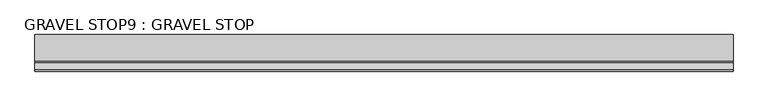
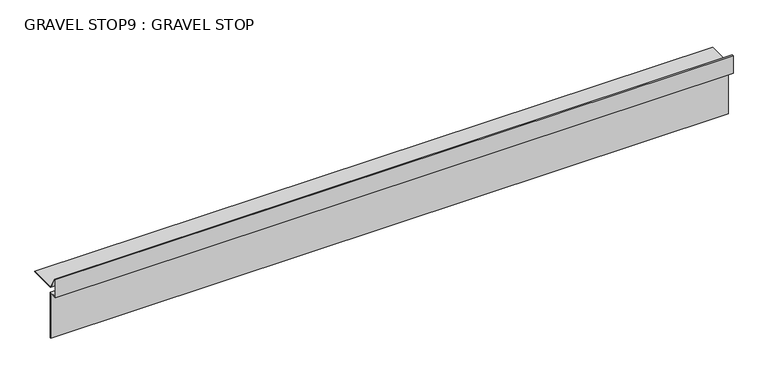
"""IFC4 building model written with IfcOpenShell, lengths in millimetres: proxy geometry, GRAVEL STOP9 : GRAVEL STOP."""

import ifcopenshell
import ifcopenshell.guid

model = None  # the IFC model being written
_history = None  # IfcOwnerHistory: only IFC2X3 demands one
_inside = {}  # id of a spatial element -> (the spatial element, [elements in it])
_under = {}  # id of a project, library or spatial element -> (it, [spatial elements below it])
_declared = {}  # id of a project -> (the project, [libraries it declares])
_typed = {}  # id of a type object -> (the type object, [elements of that type])
_made_of = {}  # id of a material, layer set ... -> (it, [elements and type objects made of it])


def new_model(schema):
    """Start an empty IFC model of exactly this schema.

    Asked for "IFC4X3", IfcOpenShell would pick the latest addendum, in which some entities
    have other attributes; the version numbers below select the first issue.
    IFC2X3 requires an IfcOwnerHistory on every rooted entity: one is made here for all.
    """
    global model, _history
    if schema == "IFC4X3":
        model = ifcopenshell.file(schema_version=(4, 3, 0, 0))
    else:
        model = ifcopenshell.file(schema=schema)
    _inside.clear()
    _under.clear()
    _declared.clear()
    _typed.clear()
    _made_of.clear()
    _history = None
    if model.schema == "IFC2X3":
        org = make("IfcOrganization", Name="unknown")
        user = make(
            "IfcPersonAndOrganization",
            ThePerson=make("IfcPerson", FamilyName="unknown"),
            TheOrganization=org,
        )
        app = make(
            "IfcApplication",
            ApplicationDeveloper=org,
            Version="unknown",
            ApplicationFullName="unknown",
            ApplicationIdentifier="unknown",
        )
        _history = make(
            "IfcOwnerHistory",
            OwningUser=user,
            OwningApplication=app,
            ChangeAction="ADDED",
            CreationDate=0,
        )
    return model


def make(cls, **values):
    """One entity of the class cls with the attributes given. An attribute that is None is left unset."""
    return model.create_entity(
        cls, **{name: value for name, value in values.items() if value is not None}
    )


def rooted(cls, **values):
    """An entity with a GlobalId (a new one), such as an element, a storey or a relation."""
    return make(cls, GlobalId=ifcopenshell.guid.new(), OwnerHistory=_history, **values)


def si_unit(unit_type, name, prefix=None):
    """IfcSIUnit, for example si_unit("LENGTHUNIT", "METRE", prefix="MILLI")."""
    return make("IfcSIUnit", UnitType=unit_type, Prefix=prefix, Name=name)


def assignment(units):
    """IfcUnitAssignment: the units of a project."""
    return None if units is None else make("IfcUnitAssignment", Units=units)


def point(xyz):
    """IfcCartesianPoint."""
    return None if xyz is None else make("IfcCartesianPoint", Coordinates=xyz)


def direction(xyz):
    """IfcDirection."""
    return None if xyz is None else make("IfcDirection", DirectionRatios=xyz)


def frame(location, z_axis=None, x_axis=None):
    """IfcAxis2Placement3D, a coordinate frame: its origin and axes. An axis left out is left unset."""
    return make(
        "IfcAxis2Placement3D",
        Location=point(location),
        Axis=direction(z_axis),
        RefDirection=direction(x_axis),
    )


def origin():
    """The frame at (0, 0, 0) with its axes left unset."""
    return frame((0.0, 0.0, 0.0))


def place(relative_to, where):
    """IfcLocalPlacement: puts the frame where relative to a parent placement (None: the world)."""
    return make(
        "IfcLocalPlacement", PlacementRelTo=relative_to, RelativePlacement=where
    )


def context(
    kind, dimensions, precision=None, world=None, true_north=None, identifier=None
):
    """IfcGeometricRepresentationContext, for example the 3D "Model" context."""
    return make(
        "IfcGeometricRepresentationContext",
        ContextIdentifier=identifier,
        ContextType=kind,
        CoordinateSpaceDimension=dimensions,
        Precision=precision,
        WorldCoordinateSystem=world,
        TrueNorth=true_north,
    )


def project(units=None, contexts=None):
    """IfcProject with its units and contexts."""
    return rooted(
        "IfcProject",
        Name="project",
        RepresentationContexts=contexts,
        UnitsInContext=assignment(units),
    )


def spatial(cls, under=None, at=None, **own):
    """A site, building, storey or space (cls), placed at a placement, below another one or the project."""
    s = rooted(cls, ObjectPlacement=at, **own)
    if under is not None:
        _under.setdefault(under.id(), (under, []))[1].append(s)
    return s


def polyline(points):
    """IfcPolyline through the points."""
    return make("IfcPolyline", Points=[point(p) for p in points])


def outline(outer, holes=None, kind="AREA"):
    """IfcArbitraryClosedProfileDef: a profile drawn as a closed curve; with holes, ...WithVoids."""
    if holes is None:
        return make("IfcArbitraryClosedProfileDef", ProfileType=kind, OuterCurve=outer)
    return make(
        "IfcArbitraryProfileDefWithVoids",
        ProfileType=kind,
        OuterCurve=outer,
        InnerCurves=holes,
    )


def extrude(swept, where, along, depth):
    """IfcExtrudedAreaSolid: the profile swept, set in the frame where, extruded along a direction by depth."""
    return make(
        "IfcExtrudedAreaSolid",
        SweptArea=swept,
        Position=where,
        ExtrudedDirection=direction(along),
        Depth=depth,
    )


def shape(context_of_items, identifier, shape_type, items):
    """IfcShapeRepresentation: the items that make up one representation, for example the "Body"."""
    return make(
        "IfcShapeRepresentation",
        ContextOfItems=context_of_items,
        RepresentationIdentifier=identifier,
        RepresentationType=shape_type,
        Items=items,
    )


def source(mapping_origin, context_of_items, identifier, shape_type, items):
    """IfcRepresentationMap: a shape defined once, which mapped items show again and again."""
    return make(
        "IfcRepresentationMap",
        MappingOrigin=mapping_origin,
        MappedRepresentation=shape(context_of_items, identifier, shape_type, items),
    )


def transform(
    local_origin,
    x_axis=None,
    y_axis=None,
    z_axis=None,
    scale=None,
    scale2=None,
    scale3=None,
    uniform=True,
):
    """IfcCartesianTransformationOperator3D, or its non-uniform kind. x_axis, y_axis, z_axis: its Axis1, 2, 3."""
    if uniform:
        return make(
            "IfcCartesianTransformationOperator3D",
            Axis1=direction(x_axis),
            Axis2=direction(y_axis),
            LocalOrigin=point(local_origin),
            Scale=scale,
            Axis3=direction(z_axis),
        )
    return make(
        "IfcCartesianTransformationOperator3DnonUniform",
        Axis1=direction(x_axis),
        Axis2=direction(y_axis),
        LocalOrigin=point(local_origin),
        Scale=scale,
        Axis3=direction(z_axis),
        Scale2=scale2,
        Scale3=scale3,
    )


def mapped(mapping_source, mapping_target):
    """IfcMappedItem: shows the shape of a source again, moved by a transform."""
    return make(
        "IfcMappedItem", MappingSource=mapping_source, MappingTarget=mapping_target
    )


def made_of(thing, what):
    """Note that an element or type object is made of a material, layer set ...; save() writes the relation."""
    if what is not None:
        _made_of.setdefault(what.id(), (what, []))[1].append(thing)
    return thing


def element(
    cls,
    number,
    at=None,
    inside=None,
    cuts=None,
    type_object=None,
    material=None,
    context=None,
    identifier="Body",
    shape_type=None,
    held_by="IfcProductDefinitionShape",
    body=None,
    shapes=None,
    **own,
):
    """One element of the class cls, such as IfcWall. Its Tag is "e" and its number.

    at: its placement. inside: the storey or other place that contains it. cuts: it is an
    opening in that element (IfcRelVoidsElement). A single representation is given by context,
    identifier, shape_type and body (its items); several are given by shapes. held_by: the class
    of the entity that holds the representations. save() writes the other relations.
    """
    e = rooted(cls, Tag="e%d" % number, ObjectPlacement=at, **own)
    if body is not None:
        shapes = [shape(context, identifier, shape_type, body)]
    if shapes is not None:
        e.Representation = make(held_by, Representations=shapes)
    if inside is not None:
        _inside.setdefault(inside.id(), (inside, []))[1].append(e)
    if cuts is not None:
        rooted(
            "IfcRelVoidsElement", RelatingBuildingElement=cuts, RelatedOpeningElement=e
        )
    if type_object is not None:
        _typed.setdefault(type_object.id(), (type_object, []))[1].append(e)
    return made_of(e, material)


def aggregate(whole, parts):
    """IfcRelAggregates: a whole, such as a stair, and the parts it consists of."""
    return rooted("IfcRelAggregates", RelatingObject=whole, RelatedObjects=parts)


def save(model, path):
    """Write the relations noted so far, then the file.

    IfcRelAggregates (storeys below a building ...), IfcRelContainedInSpatialStructure (elements
    in a storey), IfcRelDefinesByType, IfcRelAssociatesMaterial and IfcRelDeclares: one each for
    every whole, place, type object, material and project.
    """
    for whole, parts in _under.values():
        aggregate(whole, parts)
    for where, things in _inside.values():
        rooted(
            "IfcRelContainedInSpatialStructure",
            RelatedElements=things,
            RelatingStructure=where,
        )
    for kind, things in _typed.values():
        rooted("IfcRelDefinesByType", RelatedObjects=things, RelatingType=kind)
    for what, things in _made_of.values():
        rooted("IfcRelAssociatesMaterial", RelatedObjects=things, RelatingMaterial=what)
    for by, libraries in _declared.values():
        rooted("IfcRelDeclares", RelatingContext=by, RelatedDefinitions=libraries)
    model.write(path)


def gravel_stop9_gravel_stop_f17445ac(model_context):
    return source(origin(), model_context, "Body", "SweptSolid", [
        extrude(outline(polyline([(-5580.0356381, 40278.1940248), (-5577.0037237, 40279.0064238), (-5556.3332702, 40243.204148), (-5552.58096, 40241.0377507), (-5475.1230533, 40241.0377507), (-5475.1230533, 40239.6266397), (-5552.959066, 40239.6266397), (-5557.3662751, 40242.1711431), (-5577.6843899, 40277.3631503), (-5578.6245271, 40277.1112413), (-5578.6245271, 40224.6266397), (-5554.2847895, 40224.6266397), (-5554.2847895, 40081.6491197), (-5555.6959005, 40081.6491197), (-5555.6959005, 40223.2155287), (-5580.0356381, 40223.2155287), (-5580.0356381, 40278.1940248)])), frame((12382.7678845, 0.0, 0.0), z_axis=(1.0, 0.0, 0.0), x_axis=(0.0, 1.0, 0.0)), (0.0, 0.0, 1.0), 2000.25),
    ])


if __name__ == "__main__":
    model = new_model("IFC4")
    model_context = context("Model", 3, world=origin())
    ifc_project = project(units=[si_unit("LENGTHUNIT", "METRE", prefix="MILLI")], contexts=[model_context])
    site = spatial("IfcSite", under=ifc_project)
    building = spatial("IfcBuilding", under=site)
    placement = place(None, origin())
    gravel_stop9_gravel_stop_shape = gravel_stop9_gravel_stop_f17445ac(model_context)
    element("IfcBuildingElementProxy", 1, Name="GRAVEL STOP9 : GRAVEL STOP", ObjectType="GRAVEL STOP9 : GRAVEL STOP", at=placement, inside=building, context=model_context, shape_type="MappedRepresentation", body=[
        mapped(gravel_stop9_gravel_stop_shape, transform((0.0, 0.0, 0.0), x_axis=(1.0, 0.0, 0.0), y_axis=(0.0, 1.0, 0.0), z_axis=(0.0, 0.0, 1.0))),
    ])
    save(model, "model.ifc")

# Revit data of these elements
# Type "GRAVEL STOP9 : GRAVEL STOP"
#   NameOverride = "GRAVEL STOP"
# Element 1 (IfcBuildingElementProxy, "GRAVEL STOP9 : GRAVEL STOP")
#   Materials on its faces: "GRAVEL STOP REQUIRED WITH GRAVEL SURFACE SYSTEMS"
# Materials
#   "GRAVEL STOP REQUIRED WITH GRAVEL SURFACE SYSTEMS": class "Unassigned", colour RGB 170 170 127, transparency 0, Cost = 0
